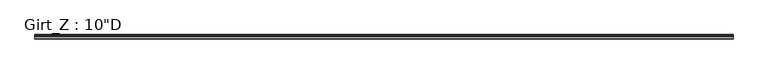
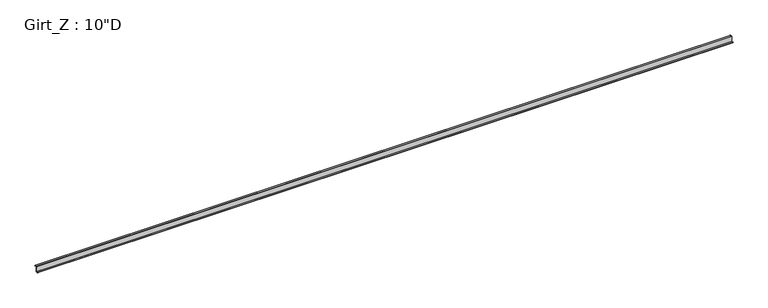
"""IFC4 building model written with IfcOpenShell, lengths in millimetres: beam geometry."""

import ifcopenshell
import ifcopenshell.guid

model = None  # the IFC model being written
_history = None  # IfcOwnerHistory: only IFC2X3 demands one
_inside = {}  # id of a spatial element -> (the spatial element, [elements in it])
_under = {}  # id of a project, library or spatial element -> (it, [spatial elements below it])
_declared = {}  # id of a project -> (the project, [libraries it declares])
_typed = {}  # id of a type object -> (the type object, [elements of that type])
_made_of = {}  # id of a material, layer set ... -> (it, [elements and type objects made of it])


def new_model(schema):
    """Start an empty IFC model of exactly this schema.

    Asked for "IFC4X3", IfcOpenShell would pick the latest addendum, in which some entities
    have other attributes; the version numbers below select the first issue.
    IFC2X3 requires an IfcOwnerHistory on every rooted entity: one is made here for all.
    """
    global model, _history
    if schema == "IFC4X3":
        model = ifcopenshell.file(schema_version=(4, 3, 0, 0))
    else:
        model = ifcopenshell.file(schema=schema)
    _inside.clear()
    _under.clear()
    _declared.clear()
    _typed.clear()
    _made_of.clear()
    _history = None
    if model.schema == "IFC2X3":
        org = make("IfcOrganization", Name="unknown")
        user = make(
            "IfcPersonAndOrganization",
            ThePerson=make("IfcPerson", FamilyName="unknown"),
            TheOrganization=org,
        )
        app = make(
            "IfcApplication",
            ApplicationDeveloper=org,
            Version="unknown",
            ApplicationFullName="unknown",
            ApplicationIdentifier="unknown",
        )
        _history = make(
            "IfcOwnerHistory",
            OwningUser=user,
            OwningApplication=app,
            ChangeAction="ADDED",
            CreationDate=0,
        )
    return model


def make(cls, **values):
    """One entity of the class cls with the attributes given. An attribute that is None is left unset."""
    return model.create_entity(
        cls, **{name: value for name, value in values.items() if value is not None}
    )


def rooted(cls, **values):
    """An entity with a GlobalId (a new one), such as an element, a storey or a relation."""
    return make(cls, GlobalId=ifcopenshell.guid.new(), OwnerHistory=_history, **values)


def si_unit(unit_type, name, prefix=None):
    """IfcSIUnit, for example si_unit("LENGTHUNIT", "METRE", prefix="MILLI")."""
    return make("IfcSIUnit", UnitType=unit_type, Prefix=prefix, Name=name)


def assignment(units):
    """IfcUnitAssignment: the units of a project."""
    return None if units is None else make("IfcUnitAssignment", Units=units)


def point(xyz):
    """IfcCartesianPoint."""
    return None if xyz is None else make("IfcCartesianPoint", Coordinates=xyz)


def direction(xyz):
    """IfcDirection."""
    return None if xyz is None else make("IfcDirection", DirectionRatios=xyz)


def frame(location, z_axis=None, x_axis=None):
    """IfcAxis2Placement3D, a coordinate frame: its origin and axes. An axis left out is left unset."""
    return make(
        "IfcAxis2Placement3D",
        Location=point(location),
        Axis=direction(z_axis),
        RefDirection=direction(x_axis),
    )


def frame_2d(location, x_axis=None):
    """IfcAxis2Placement2D, a coordinate frame in the plane: its origin and x axis."""
    return make(
        "IfcAxis2Placement2D", Location=point(location), RefDirection=direction(x_axis)
    )


def origin():
    """The frame at (0, 0, 0) with its axes left unset."""
    return frame((0.0, 0.0, 0.0))


def place(relative_to, where):
    """IfcLocalPlacement: puts the frame where relative to a parent placement (None: the world)."""
    return make(
        "IfcLocalPlacement", PlacementRelTo=relative_to, RelativePlacement=where
    )


def context(
    kind, dimensions, precision=None, world=None, true_north=None, identifier=None
):
    """IfcGeometricRepresentationContext, for example the 3D "Model" context."""
    return make(
        "IfcGeometricRepresentationContext",
        ContextIdentifier=identifier,
        ContextType=kind,
        CoordinateSpaceDimension=dimensions,
        Precision=precision,
        WorldCoordinateSystem=world,
        TrueNorth=true_north,
    )


def project(units=None, contexts=None):
    """IfcProject with its units and contexts."""
    return rooted(
        "IfcProject",
        Name="project",
        RepresentationContexts=contexts,
        UnitsInContext=assignment(units),
    )


def spatial(cls, under=None, at=None, **own):
    """A site, building, storey or space (cls), placed at a placement, below another one or the project."""
    s = rooted(cls, ObjectPlacement=at, **own)
    if under is not None:
        _under.setdefault(under.id(), (under, []))[1].append(s)
    return s


def polyline(points):
    """IfcPolyline through the points."""
    return make("IfcPolyline", Points=[point(p) for p in points])


def circle_curve(where, radius):
    """IfcCircle in the frame where."""
    return make("IfcCircle", Position=where, Radius=radius)


def trimmed(basis, trim1, trim2, sense, master):
    """IfcTrimmedCurve: the piece of a basis curve between two trims."""
    return make(
        "IfcTrimmedCurve",
        BasisCurve=basis,
        Trim1=trim1,
        Trim2=trim2,
        SenseAgreement=sense,
        MasterRepresentation=master,
    )


def segment(curve, same_sense, transition):
    """IfcCompositeCurveSegment."""
    return make(
        "IfcCompositeCurveSegment",
        Transition=transition,
        SameSense=same_sense,
        ParentCurve=curve,
    )


def composite_curve(segments, self_intersect=None):
    """IfcCompositeCurve: segments joined end to end."""
    return make("IfcCompositeCurve", Segments=segments, SelfIntersect=self_intersect)


def outline(outer, holes=None, kind="AREA"):
    """IfcArbitraryClosedProfileDef: a profile drawn as a closed curve; with holes, ...WithVoids."""
    if holes is None:
        return make("IfcArbitraryClosedProfileDef", ProfileType=kind, OuterCurve=outer)
    return make(
        "IfcArbitraryProfileDefWithVoids",
        ProfileType=kind,
        OuterCurve=outer,
        InnerCurves=holes,
    )


def extrude(swept, where, along, depth):
    """IfcExtrudedAreaSolid: the profile swept, set in the frame where, extruded along a direction by depth."""
    return make(
        "IfcExtrudedAreaSolid",
        SweptArea=swept,
        Position=where,
        ExtrudedDirection=direction(along),
        Depth=depth,
    )


def shape(context_of_items, identifier, shape_type, items):
    """IfcShapeRepresentation: the items that make up one representation, for example the "Body"."""
    return make(
        "IfcShapeRepresentation",
        ContextOfItems=context_of_items,
        RepresentationIdentifier=identifier,
        RepresentationType=shape_type,
        Items=items,
    )


def source(mapping_origin, context_of_items, identifier, shape_type, items):
    """IfcRepresentationMap: a shape defined once, which mapped items show again and again."""
    return make(
        "IfcRepresentationMap",
        MappingOrigin=mapping_origin,
        MappedRepresentation=shape(context_of_items, identifier, shape_type, items),
    )


def transform(
    local_origin,
    x_axis=None,
    y_axis=None,
    z_axis=None,
    scale=None,
    scale2=None,
    scale3=None,
    uniform=True,
):
    """IfcCartesianTransformationOperator3D, or its non-uniform kind. x_axis, y_axis, z_axis: its Axis1, 2, 3."""
    if uniform:
        return make(
            "IfcCartesianTransformationOperator3D",
            Axis1=direction(x_axis),
            Axis2=direction(y_axis),
            LocalOrigin=point(local_origin),
            Scale=scale,
            Axis3=direction(z_axis),
        )
    return make(
        "IfcCartesianTransformationOperator3DnonUniform",
        Axis1=direction(x_axis),
        Axis2=direction(y_axis),
        LocalOrigin=point(local_origin),
        Scale=scale,
        Axis3=direction(z_axis),
        Scale2=scale2,
        Scale3=scale3,
    )


def mapped(mapping_source, mapping_target):
    """IfcMappedItem: shows the shape of a source again, moved by a transform."""
    return make(
        "IfcMappedItem", MappingSource=mapping_source, MappingTarget=mapping_target
    )


def made_of(thing, what):
    """Note that an element or type object is made of a material, layer set ...; save() writes the relation."""
    if what is not None:
        _made_of.setdefault(what.id(), (what, []))[1].append(thing)
    return thing


def element(
    cls,
    number,
    at=None,
    inside=None,
    cuts=None,
    type_object=None,
    material=None,
    context=None,
    identifier="Body",
    shape_type=None,
    held_by="IfcProductDefinitionShape",
    body=None,
    shapes=None,
    **own,
):
    """One element of the class cls, such as IfcWall. Its Tag is "e" and its number.

    at: its placement. inside: the storey or other place that contains it. cuts: it is an
    opening in that element (IfcRelVoidsElement). A single representation is given by context,
    identifier, shape_type and body (its items); several are given by shapes. held_by: the class
    of the entity that holds the representations. save() writes the other relations.
    """
    e = rooted(cls, Tag="e%d" % number, ObjectPlacement=at, **own)
    if body is not None:
        shapes = [shape(context, identifier, shape_type, body)]
    if shapes is not None:
        e.Representation = make(held_by, Representations=shapes)
    if inside is not None:
        _inside.setdefault(inside.id(), (inside, []))[1].append(e)
    if cuts is not None:
        rooted(
            "IfcRelVoidsElement", RelatingBuildingElement=cuts, RelatedOpeningElement=e
        )
    if type_object is not None:
        _typed.setdefault(type_object.id(), (type_object, []))[1].append(e)
    return made_of(e, material)


def aggregate(whole, parts):
    """IfcRelAggregates: a whole, such as a stair, and the parts it consists of."""
    return rooted("IfcRelAggregates", RelatingObject=whole, RelatedObjects=parts)


def save(model, path):
    """Write the relations noted so far, then the file.

    IfcRelAggregates (storeys below a building ...), IfcRelContainedInSpatialStructure (elements
    in a storey), IfcRelDefinesByType, IfcRelAssociatesMaterial and IfcRelDeclares: one each for
    every whole, place, type object, material and project.
    """
    for whole, parts in _under.values():
        aggregate(whole, parts)
    for where, things in _inside.values():
        rooted(
            "IfcRelContainedInSpatialStructure",
            RelatedElements=things,
            RelatingStructure=where,
        )
    for kind, things in _typed.values():
        rooted("IfcRelDefinesByType", RelatedObjects=things, RelatingType=kind)
    for what, things in _made_of.values():
        rooted("IfcRelAssociatesMaterial", RelatedObjects=things, RelatingMaterial=what)
    for by, libraries in _declared.values():
        rooted("IfcRelDeclares", RelatingContext=by, RelatedDefinitions=libraries)
    model.write(path)


def beam_638428f9(model_context):
    return source(origin(), model_context, "Body", "SweptSolid", [
        extrude(outline(composite_curve([segment(polyline([(77.9859375, 127.0), (90.2310415, 112.4068534), (88.1028742, 110.621109), (76.6904765, 124.221875), (3.3005807, 124.221875)]), True, "CONTINUOUS"), segment(trimmed(circle_curve(frame_2d((3.3741066, 122.2381931)), 1.9850441), [point((3.3005807, 124.221875))], [point((1.3890625, 122.2381931))], True, "CARTESIAN"), True, "CONTINUOUS"), segment(polyline([(1.3890625, 122.2381931), (1.3890625, -127.0), (-84.3359375, -127.0), (-96.5810415, -112.4068534), (-94.4528742, -110.621109), (-83.0404765, -124.221875), (-3.2694106, -124.221875)]), True, "CONTINUOUS"), segment(trimmed(circle_curve(frame_2d((-3.3748024, -122.2389339)), 1.9857399), [point((-3.2694106, -124.221875))], [point((-1.3890625, -122.2389339))], True, "CARTESIAN"), True, "CONTINUOUS"), segment(polyline([(-1.3890625, -122.2389339), (-1.3890625, 122.2375)]), True, "CONTINUOUS"), segment(trimmed(circle_curve(frame_2d((3.3734375, 122.2375)), 4.7625), [point((-1.3890625, 122.2375))], [point((3.3734375, 127.0))], False, "CARTESIAN"), True, "CONTINUOUS"), segment(polyline([(3.3734375, 127.0), (77.9859375, 127.0)]), True, "CONTINUOUS")], self_intersect=False)), frame((-15640.05, 0.0, 0.0), z_axis=(1.0, 0.0, 0.0), x_axis=(0.0, 1.0, 0.0)), (0.0, 0.0, 1.0), 31121.35),
    ])


if __name__ == "__main__":
    model = new_model("IFC4")
    model_context = context("Model", 3, world=origin())
    ifc_project = project(units=[si_unit("LENGTHUNIT", "METRE", prefix="MILLI")], contexts=[model_context])
    site = spatial("IfcSite", under=ifc_project)
    building = spatial("IfcBuilding", under=site)
    placement = place(None, origin())
    beam_shape = beam_638428f9(model_context)
    element("IfcBeam", 1, ObjectType="Girt_Z : 10\"D", at=placement, inside=building, context=model_context, shape_type="MappedRepresentation", body=[
        mapped(beam_shape, transform((0.0, 0.0, 0.0), x_axis=(1.0, 0.0, 0.0), y_axis=(0.0, 1.0, 0.0), z_axis=(0.0, 0.0, 1.0))),
    ])
    save(model, "model.ifc")

# Revit data of these elements
# Type "Girt_Z : 10\"D"
#   half leg = 0' - 1 11/16"
#   Web_Thickness = 0' - 0 7/64"
#   Length [instance default] = 10' - 0"
#   Leg_2 = 0' - 3 3/8"
#   Leg_1 = 0' - 3 1/8"
#   Height = 0' - 10"
#   Structural Material [instance default] = none
# Element 1 (IfcBeam, "Girt_Z : 10\"D")
#   Structural Material = STRUCTURAL STEEL - SEE STRUCT. DWGS
#   Materials on its faces: "STRUCTURAL STEEL - SEE STRUCT. DWGS"
# Materials
#   "STRUCTURAL STEEL - SEE STRUCT. DWGS": class "Metal", colour RGB 137 146 153, transparency 0, Description = "Steel, mill finish", Cost = 0
